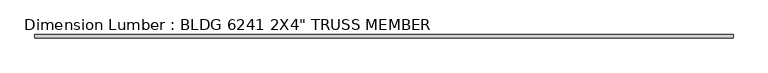
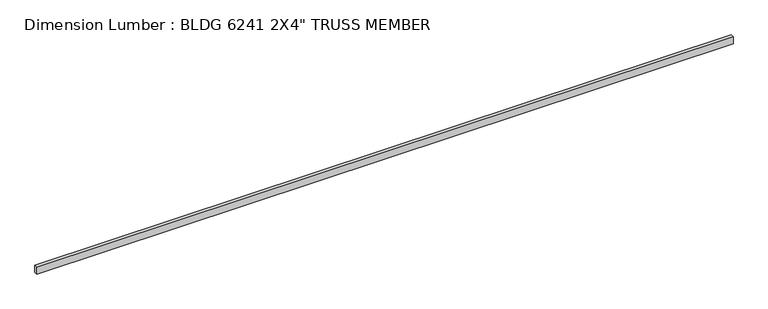
"""IFC4 building model written with IfcOpenShell, lengths in millimetres: beam geometry."""

from ifc_helpers import new_model, si_unit, frame, origin, place, context, project, spatial, polyline, outline, extrude, source, transform, mapped, element, save


def beam_8f11d8aa(model_context):
    return source(origin(), model_context, "Body", "SweptSolid", [
        extrude(outline(polyline([(5054.5999994, 25.4), (5054.5999994, -25.4), (-5054.5999994, -25.4), (-5054.5999994, 25.4), (5054.5999994, 25.4)])), frame((0.0, 0.0, -50.8), z_axis=(0.0, 0.0, 1.0), x_axis=(1.0, 0.0, 0.0)), (0.0, 0.0, 1.0), 101.6),
    ])


if __name__ == "__main__":
    model = new_model("IFC4")
    model_context = context("Model", 3, world=origin())
    ifc_project = project(units=[si_unit("LENGTHUNIT", "METRE", prefix="MILLI")], contexts=[model_context])
    site = spatial("IfcSite", under=ifc_project)
    building = spatial("IfcBuilding", under=site)
    placement = place(None, origin())
    beam_shape = beam_8f11d8aa(model_context)
    element("IfcBeam", 1, ObjectType="Dimension Lumber : BLDG 6241 2X4\" TRUSS MEMBER", at=placement, inside=building, context=model_context, shape_type="MappedRepresentation", body=[
        mapped(beam_shape, transform((0.0, 0.0, 0.0), x_axis=(1.0, 0.0, 0.0), y_axis=(0.0, 1.0, 0.0), z_axis=(0.0, 0.0, 1.0))),
    ])
    save(model, "model.ifc")

# Revit data of these elements
# Type "Dimension Lumber : BLDG 6241 2X4\" TRUSS MEMBER"
#   Assembly Code = "B10"
#   A = 0.273472 SF
#   Length [instance default] = 5' - 0"
#   b = 0' - 2"
#   d = 0' - 4"
#   Structural Material [instance default] = Softwood, Lumber
# Element 1 (IfcBeam, "Dimension Lumber : BLDG 6241 2X4\" TRUSS MEMBER")
#   Materials on its faces: "Softwood, Lumber"
# Materials
#   "Softwood, Lumber": class "Wood", colour RGB 223 192 134, transparency 0, Description = "Pinus Echinata", Cost = 0
